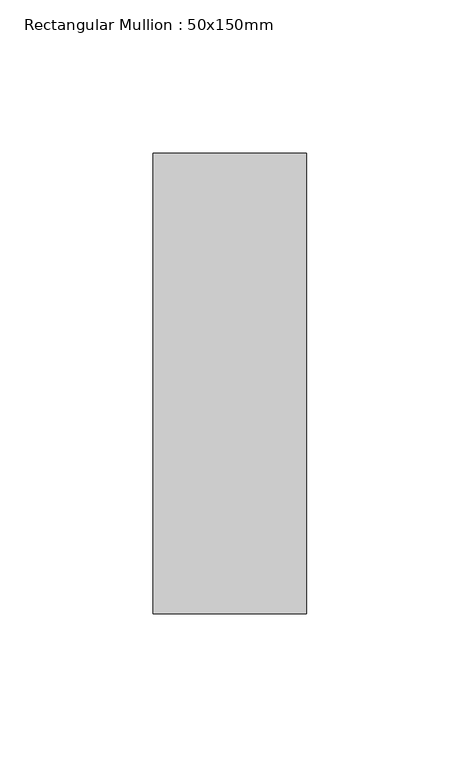
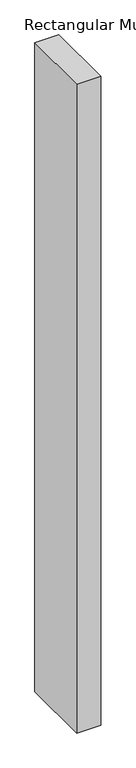
"""IFC4 building model written with IfcOpenShell, lengths in millimetres: member geometry, Rectangular Mullion : 50x150mm."""

from ifc_helpers import new_model, si_unit, frame, origin, place, context, project, spatial, polyline, outline, extrude, source, transform, mapped, element, save


def rectangular_mullion_50x150mm_751a5dca(model_context):
    return source(origin(), model_context, "Body", "SweptSolid", [
        extrude(outline(polyline([(0.0, 75.0), (0.0, -75.0), (-50.0, -75.0), (-50.0, 75.0), (0.0, 75.0)])), frame((0.0, 0.0, -1425.0), z_axis=(0.0, 0.0, 1.0), x_axis=(1.0, 0.0, 0.0)), (0.0, 0.0, 1.0), 1425.0),
    ])


if __name__ == "__main__":
    model = new_model("IFC4")
    model_context = context("Model", 3, world=origin())
    ifc_project = project(units=[si_unit("LENGTHUNIT", "METRE", prefix="MILLI")], contexts=[model_context])
    site = spatial("IfcSite", under=ifc_project)
    building = spatial("IfcBuilding", under=site)
    placement = place(None, origin())
    rectangular_mullion_50x150mm_shape = rectangular_mullion_50x150mm_751a5dca(model_context)
    element("IfcMember", 1, ObjectType="Rectangular Mullion : 50x150mm", at=placement, inside=building, context=model_context, shape_type="MappedRepresentation", body=[
        mapped(rectangular_mullion_50x150mm_shape, transform((0.0, 0.0, 0.0), x_axis=(1.0, 0.0, 0.0), y_axis=(0.0, 1.0, 0.0), z_axis=(0.0, 0.0, 1.0))),
    ])
    save(model, "model.ifc")

# Revit data of these elements
# Type "Rectangular Mullion : 50x150mm"
#   Keynote = "H11"
#   built-in parameter 1007304 = 0.492126 (stored number, unit not read)
#   built-in parameter 1007301 = 0.082021 (stored number, unit not read)
#   built-in parameter 1007300 = 0.082021 (stored number, unit not read)
# Element 1 (IfcMember, "Rectangular Mullion : 50x150mm")
#   Materials on its faces: "Aluminium"
# Materials
#   "Aluminium": class "Metal", colour RGB 247 247 247, transparency 0, Description = "Aluminium 6061", Cost = 0
